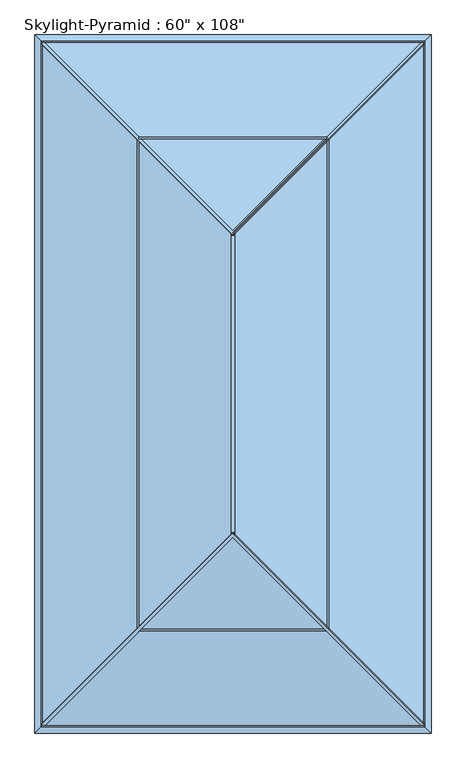
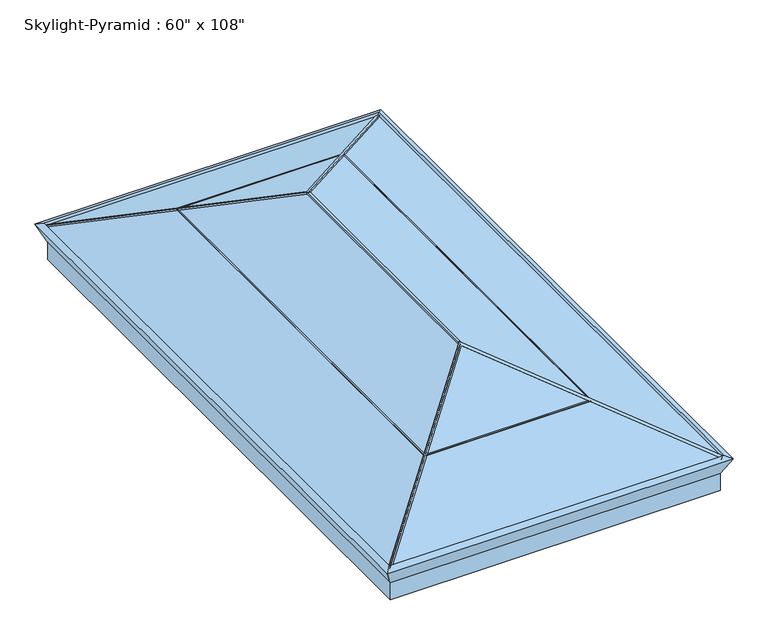
"""IFC4 building model written with IfcOpenShell, lengths in millimetres: window geometry."""

import ifcopenshell
import ifcopenshell.guid

model = None  # the IFC model being written
_history = None  # IfcOwnerHistory: only IFC2X3 demands one
_inside = {}  # id of a spatial element -> (the spatial element, [elements in it])
_under = {}  # id of a project, library or spatial element -> (it, [spatial elements below it])
_declared = {}  # id of a project -> (the project, [libraries it declares])
_typed = {}  # id of a type object -> (the type object, [elements of that type])
_made_of = {}  # id of a material, layer set ... -> (it, [elements and type objects made of it])


def new_model(schema):
    """Start an empty IFC model of exactly this schema.

    Asked for "IFC4X3", IfcOpenShell would pick the latest addendum, in which some entities
    have other attributes; the version numbers below select the first issue.
    IFC2X3 requires an IfcOwnerHistory on every rooted entity: one is made here for all.
    """
    global model, _history
    if schema == "IFC4X3":
        model = ifcopenshell.file(schema_version=(4, 3, 0, 0))
    else:
        model = ifcopenshell.file(schema=schema)
    _inside.clear()
    _under.clear()
    _declared.clear()
    _typed.clear()
    _made_of.clear()
    _history = None
    if model.schema == "IFC2X3":
        org = make("IfcOrganization", Name="unknown")
        user = make(
            "IfcPersonAndOrganization",
            ThePerson=make("IfcPerson", FamilyName="unknown"),
            TheOrganization=org,
        )
        app = make(
            "IfcApplication",
            ApplicationDeveloper=org,
            Version="unknown",
            ApplicationFullName="unknown",
            ApplicationIdentifier="unknown",
        )
        _history = make(
            "IfcOwnerHistory",
            OwningUser=user,
            OwningApplication=app,
            ChangeAction="ADDED",
            CreationDate=0,
        )
    return model


def make(cls, **values):
    """One entity of the class cls with the attributes given. An attribute that is None is left unset."""
    return model.create_entity(
        cls, **{name: value for name, value in values.items() if value is not None}
    )


def rooted(cls, **values):
    """An entity with a GlobalId (a new one), such as an element, a storey or a relation."""
    return make(cls, GlobalId=ifcopenshell.guid.new(), OwnerHistory=_history, **values)


def si_unit(unit_type, name, prefix=None):
    """IfcSIUnit, for example si_unit("LENGTHUNIT", "METRE", prefix="MILLI")."""
    return make("IfcSIUnit", UnitType=unit_type, Prefix=prefix, Name=name)


def assignment(units):
    """IfcUnitAssignment: the units of a project."""
    return None if units is None else make("IfcUnitAssignment", Units=units)


def point(xyz):
    """IfcCartesianPoint."""
    return None if xyz is None else make("IfcCartesianPoint", Coordinates=xyz)


def direction(xyz):
    """IfcDirection."""
    return None if xyz is None else make("IfcDirection", DirectionRatios=xyz)


def frame(location, z_axis=None, x_axis=None):
    """IfcAxis2Placement3D, a coordinate frame: its origin and axes. An axis left out is left unset."""
    return make(
        "IfcAxis2Placement3D",
        Location=point(location),
        Axis=direction(z_axis),
        RefDirection=direction(x_axis),
    )


def origin():
    """The frame at (0, 0, 0) with its axes left unset."""
    return frame((0.0, 0.0, 0.0))


def place(relative_to, where):
    """IfcLocalPlacement: puts the frame where relative to a parent placement (None: the world)."""
    return make(
        "IfcLocalPlacement", PlacementRelTo=relative_to, RelativePlacement=where
    )


def context(
    kind, dimensions, precision=None, world=None, true_north=None, identifier=None
):
    """IfcGeometricRepresentationContext, for example the 3D "Model" context."""
    return make(
        "IfcGeometricRepresentationContext",
        ContextIdentifier=identifier,
        ContextType=kind,
        CoordinateSpaceDimension=dimensions,
        Precision=precision,
        WorldCoordinateSystem=world,
        TrueNorth=true_north,
    )


def project(units=None, contexts=None):
    """IfcProject with its units and contexts."""
    return rooted(
        "IfcProject",
        Name="project",
        RepresentationContexts=contexts,
        UnitsInContext=assignment(units),
    )


def spatial(cls, under=None, at=None, **own):
    """A site, building, storey or space (cls), placed at a placement, below another one or the project."""
    s = rooted(cls, ObjectPlacement=at, **own)
    if under is not None:
        _under.setdefault(under.id(), (under, []))[1].append(s)
    return s


def polyline(points):
    """IfcPolyline through the points."""
    return make("IfcPolyline", Points=[point(p) for p in points])


def outline(outer, holes=None, kind="AREA"):
    """IfcArbitraryClosedProfileDef: a profile drawn as a closed curve; with holes, ...WithVoids."""
    if holes is None:
        return make("IfcArbitraryClosedProfileDef", ProfileType=kind, OuterCurve=outer)
    return make(
        "IfcArbitraryProfileDefWithVoids",
        ProfileType=kind,
        OuterCurve=outer,
        InnerCurves=holes,
    )


def extrude(swept, where, along, depth):
    """IfcExtrudedAreaSolid: the profile swept, set in the frame where, extruded along a direction by depth."""
    return make(
        "IfcExtrudedAreaSolid",
        SweptArea=swept,
        Position=where,
        ExtrudedDirection=direction(along),
        Depth=depth,
    )


def faces_of(points, faces, orient=None, outer=None):
    """IfcFace entities. A face is a list of loops; a loop is a list of indices into points, from 0.

    orient and outer hold one flag for each loop. By default every Orientation is true, the
    first loop of a face is its IfcFaceOuterBound and the others are IfcFaceBound.
    """
    made = []
    for i, loops in enumerate(faces):
        bounds = []
        for j, loop in enumerate(loops):
            is_outer = j == 0 if outer is None else outer[i][j]
            bounds.append(
                make(
                    "IfcFaceOuterBound" if is_outer else "IfcFaceBound",
                    Bound=make("IfcPolyLoop", Polygon=[points[k] for k in loop]),
                    Orientation=True if orient is None else orient[i][j],
                )
            )
        made.append(make("IfcFace", Bounds=bounds))
    return made


def faceted_brep(points, faces, orient=None, outer=None, voids=None):
    """IfcFacetedBrep: a solid bounded by flat faces; with voids (closed shells), ...WithVoids."""
    shared = [point(p) for p in points]
    hull = make("IfcClosedShell", CfsFaces=faces_of(shared, faces, orient, outer))
    if voids is None:
        return make("IfcFacetedBrep", Outer=hull)
    return make(
        "IfcFacetedBrepWithVoids",
        Outer=hull,
        Voids=[
            make(cls, CfsFaces=faces_of(shared, fs, o, b)) for cls, fs, o, b in voids
        ],
    )


def shape(context_of_items, identifier, shape_type, items):
    """IfcShapeRepresentation: the items that make up one representation, for example the "Body"."""
    return make(
        "IfcShapeRepresentation",
        ContextOfItems=context_of_items,
        RepresentationIdentifier=identifier,
        RepresentationType=shape_type,
        Items=items,
    )


def source(mapping_origin, context_of_items, identifier, shape_type, items):
    """IfcRepresentationMap: a shape defined once, which mapped items show again and again."""
    return make(
        "IfcRepresentationMap",
        MappingOrigin=mapping_origin,
        MappedRepresentation=shape(context_of_items, identifier, shape_type, items),
    )


def transform(
    local_origin,
    x_axis=None,
    y_axis=None,
    z_axis=None,
    scale=None,
    scale2=None,
    scale3=None,
    uniform=True,
):
    """IfcCartesianTransformationOperator3D, or its non-uniform kind. x_axis, y_axis, z_axis: its Axis1, 2, 3."""
    if uniform:
        return make(
            "IfcCartesianTransformationOperator3D",
            Axis1=direction(x_axis),
            Axis2=direction(y_axis),
            LocalOrigin=point(local_origin),
            Scale=scale,
            Axis3=direction(z_axis),
        )
    return make(
        "IfcCartesianTransformationOperator3DnonUniform",
        Axis1=direction(x_axis),
        Axis2=direction(y_axis),
        LocalOrigin=point(local_origin),
        Scale=scale,
        Axis3=direction(z_axis),
        Scale2=scale2,
        Scale3=scale3,
    )


def mapped(mapping_source, mapping_target):
    """IfcMappedItem: shows the shape of a source again, moved by a transform."""
    return make(
        "IfcMappedItem", MappingSource=mapping_source, MappingTarget=mapping_target
    )


def made_of(thing, what):
    """Note that an element or type object is made of a material, layer set ...; save() writes the relation."""
    if what is not None:
        _made_of.setdefault(what.id(), (what, []))[1].append(thing)
    return thing


def element(
    cls,
    number,
    at=None,
    inside=None,
    cuts=None,
    type_object=None,
    material=None,
    context=None,
    identifier="Body",
    shape_type=None,
    held_by="IfcProductDefinitionShape",
    body=None,
    shapes=None,
    **own,
):
    """One element of the class cls, such as IfcWall. Its Tag is "e" and its number.

    at: its placement. inside: the storey or other place that contains it. cuts: it is an
    opening in that element (IfcRelVoidsElement). A single representation is given by context,
    identifier, shape_type and body (its items); several are given by shapes. held_by: the class
    of the entity that holds the representations. save() writes the other relations.
    """
    e = rooted(cls, Tag="e%d" % number, ObjectPlacement=at, **own)
    if body is not None:
        shapes = [shape(context, identifier, shape_type, body)]
    if shapes is not None:
        e.Representation = make(held_by, Representations=shapes)
    if inside is not None:
        _inside.setdefault(inside.id(), (inside, []))[1].append(e)
    if cuts is not None:
        rooted(
            "IfcRelVoidsElement", RelatingBuildingElement=cuts, RelatedOpeningElement=e
        )
    if type_object is not None:
        _typed.setdefault(type_object.id(), (type_object, []))[1].append(e)
    return made_of(e, material)


def aggregate(whole, parts):
    """IfcRelAggregates: a whole, such as a stair, and the parts it consists of."""
    return rooted("IfcRelAggregates", RelatingObject=whole, RelatedObjects=parts)


def save(model, path):
    """Write the relations noted so far, then the file.

    IfcRelAggregates (storeys below a building ...), IfcRelContainedInSpatialStructure (elements
    in a storey), IfcRelDefinesByType, IfcRelAssociatesMaterial and IfcRelDeclares: one each for
    every whole, place, type object, material and project.
    """
    for whole, parts in _under.values():
        aggregate(whole, parts)
    for where, things in _inside.values():
        rooted(
            "IfcRelContainedInSpatialStructure",
            RelatedElements=things,
            RelatingStructure=where,
        )
    for kind, things in _typed.values():
        rooted("IfcRelDefinesByType", RelatedObjects=things, RelatingType=kind)
    for what, things in _made_of.values():
        rooted("IfcRelAssociatesMaterial", RelatedObjects=things, RelatingMaterial=what)
    for by, libraries in _declared.values():
        rooted("IfcRelDeclares", RelatingContext=by, RelatedDefinitions=libraries)
    model.write(path)


def window_740b1336(model_context):
    return source(origin(), model_context, "Body", "SolidModel", [
        extrude(outline(polyline([(758.8028832, 0.0), (758.8028832, -6.3500001), (0.0, -6.3500001), (0.0, 0.0), (758.8028832, 0.0)])), frame((379.4014416, 989.5973311, 4305.4065549), z_axis=(0.0, 0.4226182617406916, 0.9063077870366536), x_axis=(-1.0, 0.0, 0.0)), (0.0, 0.0, 1.0), 3.175),
        extrude(outline(polyline([(1978.9715236, 0.0), (1978.9715236, -6.3500001), (0.0, -6.3500001), (0.0, 0.0), (1978.9715236, 0.0)])), frame((379.9973311, -989.4857618, 4305.4065549), z_axis=(0.4226182617408064, 0.0, 0.9063077870366001), x_axis=(0.0, 1.0, 0.0)), (0.0, 0.0, 1.0), 3.175),
        extrude(outline(polyline([(1978.9715236, 0.0), (1978.9715236, -6.3499999), (0.0, -6.3499999), (0.0, 0.0), (1978.9715236, 0.0)])), frame((-380.3327844, 989.4857618, 4306.1259367), z_axis=(-0.4226182617408067, 0.0, 0.9063077870366), x_axis=(0.0, -1.0, 0.0)), (0.0, 0.0, 1.0), 1.5875),
        extrude(outline(polyline([(758.8028832, 0.0), (758.8028832, -6.3500001), (0.0, -6.3500001), (0.0, 0.0), (758.8028832, 0.0)])), frame((-379.4014416, -989.5973311, 4305.4065549), z_axis=(0.0, -0.4226182617407052, 0.9063077870366474), x_axis=(1.0, 0.0, 0.0)), (0.0, 0.0, 1.0), 3.175),
        extrude(outline(polyline([(614.2507601, 4471.6538329), (-614.2507601, 4471.6538329), (-614.2507601, 4482.1851479), (-600.5215874, 4488.5871663), (600.5215874, 4488.5871663), (614.2507601, 4482.1851479), (614.2507601, 4471.6538329)])), frame((-6.35, 0.0, 0.0), z_axis=(1.0, 0.0, 0.0), x_axis=(0.0, 1.0, 0.0)), (0.0, 0.0, 1.0), 12.7),
        extrude(outline(polyline([(0.0, -12.7), (0.0, 0.0), (1137.0838643, 0.0), (1025.5812216, 1131.603674), (1038.2200138, 1132.8490383), (1151.0967638, -12.7), (0.0, -12.7)])), frame((763.6006347, -1378.3304744, 4116.9075713), z_axis=(0.0, -0.4226182617406913, 0.9063077870366538), x_axis=(-0.6715429342378434, 0.6715429342377943, 0.3131456130149697)), (0.0, 0.0, 1.0), 10.31875),
        extrude(outline(polyline([(0.0, -12.7), (0.0, 0.0), (1137.0838643, 0.0), (1025.5812216, 1131.603674), (1038.2200138, 1132.8490383), (1151.0967638, -12.7), (0.0, -12.7)])), frame((-763.6006347, 1377.2573844, 4114.6063225), z_axis=(0.0, 0.42261826174070505, 0.9063077870366474), x_axis=(0.6715429342378264, -0.6715429342378145, 0.31314561301496247)), (0.0, 0.0, 1.0), 12.7),
        extrude(outline(polyline([(1144.090314, 0.0), (1031.9006177, -1138.5763561), (0.0, 0.0), (1144.090314, 0.0)])), frame((-768.3057665, -1375.5575938, 4121.0512976), z_axis=(0.0, -0.42261826174070527, 0.9063077870366475), x_axis=(0.6715429342378348, 0.671542934237803, 0.3131456130149692)), (0.0, 0.0, 1.0), 5.55625),
        extrude(outline(polyline([(1144.090314, 0.0), (1031.9006177, -1138.5763561), (0.0, 0.0), (1144.090314, 0.0)])), frame((768.3057665, 1375.5575938, 4121.0512976), z_axis=(0.0, 0.4226182617406916, 0.9063077870366536), x_axis=(-0.6715429342378365, -0.6715429342378046, 0.31314561301496197)), (0.0, 0.0, 1.0), 5.55625),
        faceted_brep([(-768.3057665, -1377.9057665, 4126.0869702), (-765.9575938, -1377.9057665, 4121.0512976), (-755.158559, -1377.9057665, 4126.0869702), (765.9575938, -1377.9057665, 4121.0512976), (768.3057665, -1377.9057665, 4126.0869702), (755.158559, -1377.9057665, 4126.0869702), (768.3057665, 1377.9057665, 4126.0869702), (765.9575938, 1377.9057665, 4121.0512976), (755.158559, 1377.9057665, 4126.0869702), (-765.9575938, 1377.9057665, 4121.0512976), (-768.3057665, 1377.9057665, 4126.0869702), (-755.158559, 1377.9057665, 4126.0869702), (0.0, 622.7472075, 4478.2231894), (0.0, -622.7472075, 4478.2231894), (0.0, 609.6, 4484.3538329), (0.0, -609.6, 4484.3538329)], [[[0, 1, 2]], [[3, 4, 5]], [[6, 7, 8]], [[9, 10, 11]], [[1, 0, 10, 9]], [[1, 9, 11, 12, 13, 2]], [[7, 3, 5, 13, 12, 8]], [[4, 3, 7, 6]], [[4, 6, 14, 15]], [[10, 0, 15, 14]], [[11, 10, 14, 6, 8, 12]], [[0, 2, 13, 5, 4, 15]]]),
        faceted_brep([(762.0, 1371.6, 3962.4), (762.0, 1371.6, 4044.95), (762.0, -1371.6, 4044.95), (762.0, -1371.6, 3962.4), (733.425, 1343.025, 4051.284925), (733.425, 1343.025, 3962.4), (733.425, -1343.025, 3962.4), (733.425, -1343.025, 4051.284925), (-762.0, -1371.6, 4044.95), (-762.0, -1371.6, 3962.4), (-733.425, -1343.025, 3962.4), (-733.425, -1343.025, 4051.284925), (-762.0, 1371.6, 4044.95), (-762.0, 1371.6, 3962.4), (-733.425, 1343.025, 3962.4), (-733.425, 1343.025, 4051.284925), (773.6730185, 1383.2730185, 4137.5970791), (773.6730185, -1383.2730185, 4137.5970791), (799.5707635, 1409.1707635, 4125.5207623), (799.5707635, -1409.1707635, 4125.5207623), (-773.6730185, -1383.2730185, 4137.5970791), (-799.5707635, -1409.1707635, 4125.5207623), (-773.6730185, 1383.2730185, 4137.5970791), (-799.5707635, 1409.1707635, 4125.5207623)], [[[0, 1, 2, 3]], [[4, 5, 6, 7]], [[3, 2, 8, 9]], [[7, 6, 10, 11]], [[9, 8, 12, 13]], [[11, 10, 14, 15]], [[13, 12, 1, 0]], [[3, 9, 13, 0], [5, 14, 10, 6]], [[15, 14, 5, 4]], [[16, 4, 7, 17]], [[18, 16, 17, 19]], [[1, 18, 19, 2]], [[17, 7, 11, 20]], [[19, 17, 20, 21]], [[2, 19, 21, 8]], [[20, 11, 15, 22]], [[21, 20, 22, 23]], [[8, 21, 23, 12]], [[22, 15, 4, 16]], [[23, 22, 16, 18]], [[12, 23, 18, 1]]]),
    ])


if __name__ == "__main__":
    model = new_model("IFC4")
    model_context = context("Model", 3, world=origin())
    ifc_project = project(units=[si_unit("LENGTHUNIT", "METRE", prefix="MILLI")], contexts=[model_context])
    site = spatial("IfcSite", under=ifc_project)
    building = spatial("IfcBuilding", under=site)
    placement = place(None, origin())
    window_shape = window_740b1336(model_context)
    element("IfcWindow", 1, ObjectType="Skylight-Pyramid : 60\" x 108\"", at=placement, inside=building, context=model_context, shape_type="MappedRepresentation", body=[
        mapped(window_shape, transform((0.0, 0.0, 0.0), x_axis=(1.0, 0.0, 0.0), y_axis=(0.0, 1.0, 0.0), z_axis=(0.0, 0.0, 1.0))),
    ])
    save(model, "model.ifc")

# Revit data of these elements
# Type "Skylight-Pyramid : 60\" x 108\""
#   Type Mark = "WT-16"
#   Fire Rating = "0.5h"
#   Assembly Code = "B2020100"
#   Analytic Construction = "Single-glazed windows - domestic"
#   Length 7 = 6' - 5.91226"
#   Length 6 = 2' - 5.87413"
#   Length 5 = 1' - 4.714"
#   Length 4 = 0' - 1.23091"
#   Length 3 = 2' - 6.29606"
#   Length 2 = 0' - 0.24941"
#   Length 1 = 0' - 1.47916"
#   Height 1 = 0' - 3.17208"
#   Angle Height = 1' - 5.29936"
#   Width = 5' - 0"
#   Visual Light Transmittance = 0.9
#   Thermal Resistance (R) = 0.9899 (h·ft²·°F)/BTU
#   Solar Heat Gain Coefficient = 0.86
#   Rough Width = 5' - 0 1/2"
#   Rough Height = 9' - 0 1/2"
#   Height = 9' - 0"
#   Heat Transfer Coefficient (U) = 1.0102 BTU/(h·ft²·°F)
#   Angle = 25.00°
#   Glass Panel Material = Glass
#   Frame Material = Metal - Bronze, Light Brush
# Element 1 (IfcWindow, "Skylight-Pyramid : 60\" x 108\"")
#   Materials on its faces: "Metal - Bronze, Light Brush", "Glass"
# Materials
#   "Glass": class "Glass", colour RGB 0 128 192, transparency 0.75, Description = "Soda Lime Glass", Cost = 0
#   "Metal - Bronze, Light Brush": class "Metal", colour RGB 113 80 70, transparency 0
